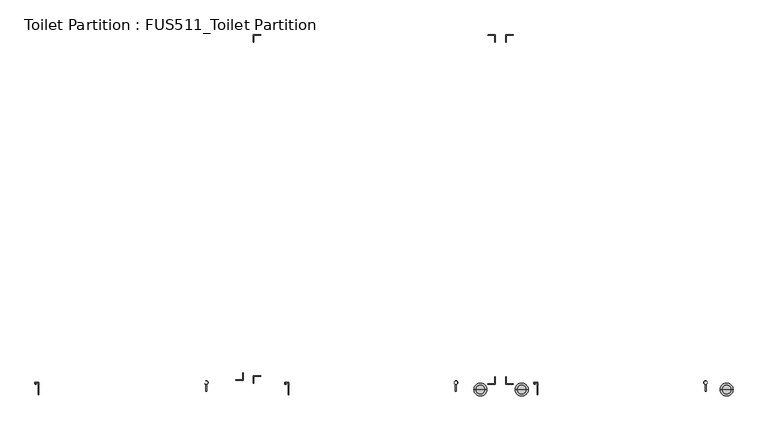
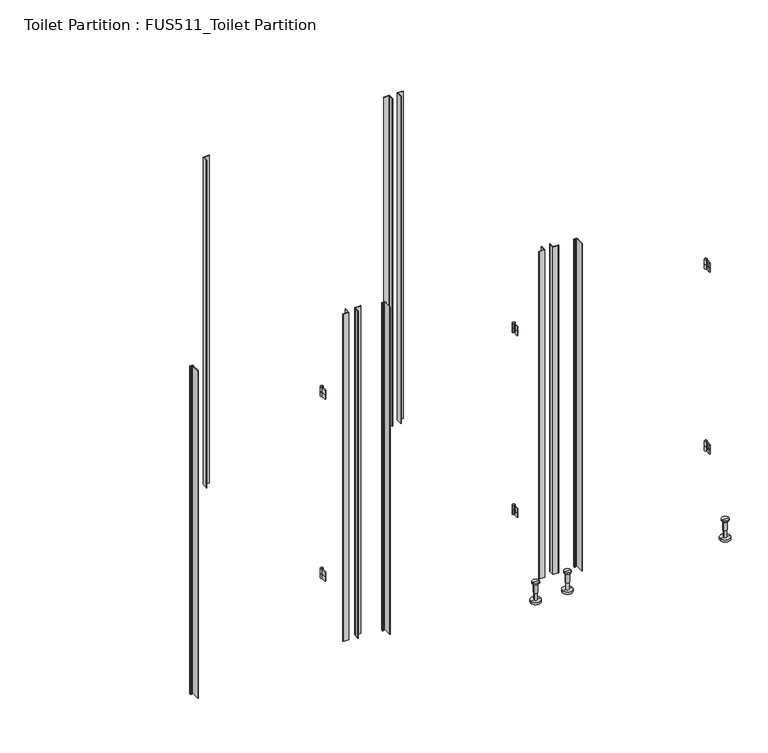
"""IFC4 building model written with IfcOpenShell, lengths in millimetres: furniture geometry, Toilet Partition : FUS511_Toilet Partition."""

from ifc_helpers import new_model, si_unit, point, frame, frame_2d, origin, place, context, project, spatial, polyline, circle_curve, trimmed, segment, composite_curve, outline, extrude, source, transform, mapped, element, save
from ifc_brep_helpers import plane_surface, cylinder_surface, advanced_brep


def toilet_partition_fus511_toilet_partition_2a8fb3a8(model_context):
    return source(origin(), model_context, "Body", "SolidModel", [
        extrude(outline(composite_curve([segment(trimmed(circle_curve(frame_2d((-483.6851629, 1892.2118377)), 1.0008364), [point((-483.6851629, 1893.2126742))], [point((-484.6859993, 1892.2118377))], True, "CARTESIAN"), True, "CONTINUOUS"), segment(polyline([(-484.6859993, 1892.2118377), (-484.6859993, 1865.1892547), (-485.6868357, 1865.1892547)]), True, "CONTINUOUS"), segment(trimmed(circle_curve(frame_2d((-485.6868357, 1866.1900911)), 1.0008364), [point((-485.6868357, 1865.1892547))], [point((-486.6876721, 1866.1900911))], False, "CARTESIAN"), True, "CONTINUOUS"), segment(polyline([(-486.6876721, 1866.1900911), (-486.6876721, 1895.214347), (-457.6634163, 1895.214347)]), True, "CONTINUOUS"), segment(trimmed(circle_curve(frame_2d((-457.6634163, 1894.2135106)), 1.0008364), [point((-457.6634163, 1895.214347))], [point((-456.6625798, 1894.2135106))], False, "CARTESIAN"), True, "CONTINUOUS"), segment(polyline([(-456.6625798, 1894.2135106), (-456.6625798, 1893.2126742), (-483.6851629, 1893.2126742)]), True, "CONTINUOUS")], self_intersect=False)), frame((0.0, 0.0, 100.0), z_axis=(0.0, 0.0, 1.0), x_axis=(1.0, 0.0, 0.0)), (0.0, 0.0, 1.0), 1800.0),
        extrude(outline(composite_curve([segment(polyline([(478.8769058, 1893.2126742), (451.8543227, 1893.2126742), (451.8543227, 1894.2135106)]), True, "CONTINUOUS"), segment(trimmed(circle_curve(frame_2d((452.8551591, 1894.2135106)), 1.0008364), [point((451.8543227, 1894.2135106))], [point((452.8551591, 1895.214347))], False, "CARTESIAN"), True, "CONTINUOUS"), segment(polyline([(452.8551591, 1895.214347), (481.879415, 1895.214347), (481.879415, 1866.1900911)]), True, "CONTINUOUS"), segment(trimmed(circle_curve(frame_2d((480.8785786, 1866.1900911)), 1.0008364), [point((481.879415, 1866.1900911))], [point((480.8785786, 1865.1892547))], False, "CARTESIAN"), True, "CONTINUOUS"), segment(polyline([(480.8785786, 1865.1892547), (479.8777422, 1865.1892547), (479.8777422, 1892.2118377)]), True, "CONTINUOUS"), segment(trimmed(circle_curve(frame_2d((478.8769058, 1892.2118377)), 1.0008364), [point((479.8777422, 1892.2118377))], [point((478.8769058, 1893.2126742))], True, "CARTESIAN"), True, "CONTINUOUS")], self_intersect=False)), frame((0.0, 0.0, 100.0), z_axis=(0.0, 0.0, 1.0), x_axis=(1.0, 0.0, 0.0)), (0.0, 0.0, 1.0), 1800.0),
        extrude(outline(composite_curve([segment(trimmed(circle_curve(frame_2d((525.8819242, 1892.2118377)), 1.0008364), [point((525.8819242, 1893.2126742))], [point((524.8810878, 1892.2118377))], True, "CARTESIAN"), True, "CONTINUOUS"), segment(polyline([(524.8810878, 1892.2118377), (524.8810878, 1865.1892547), (523.8802514, 1865.1892547)]), True, "CONTINUOUS"), segment(trimmed(circle_curve(frame_2d((523.8802514, 1866.1900911)), 1.0008364), [point((523.8802514, 1865.1892547))], [point((522.879415, 1866.1900911))], False, "CARTESIAN"), True, "CONTINUOUS"), segment(polyline([(522.879415, 1866.1900911), (522.879415, 1895.214347), (551.9036709, 1895.214347)]), True, "CONTINUOUS"), segment(trimmed(circle_curve(frame_2d((551.9036709, 1894.2135106)), 1.0008364), [point((551.9036709, 1895.214347))], [point((552.9045073, 1894.2135106))], False, "CARTESIAN"), True, "CONTINUOUS"), segment(polyline([(552.9045073, 1894.2135106), (552.9045073, 1893.2126742), (525.8819242, 1893.2126742)]), True, "CONTINUOUS")], self_intersect=False)), frame((0.0, 0.0, 100.0), z_axis=(0.0, 0.0, 1.0), x_axis=(1.0, 0.0, 0.0)), (0.0, 0.0, 1.0), 1800.0),
        extrude(outline(composite_curve([segment(trimmed(circle_curve(frame_2d((-530.6901814, 514.4572016)), 1.0008364), [point((-530.6901814, 513.4563652))], [point((-529.689345, 514.4572016))], True, "CARTESIAN"), True, "CONTINUOUS"), segment(polyline([(-529.689345, 514.4572016), (-529.689345, 541.4797847), (-528.6885085, 541.4797847)]), True, "CONTINUOUS"), segment(trimmed(circle_curve(frame_2d((-528.6885085, 540.4789483)), 1.0008364), [point((-528.6885085, 541.4797847))], [point((-527.6876721, 540.4789483))], False, "CARTESIAN"), True, "CONTINUOUS"), segment(polyline([(-527.6876721, 540.4789483), (-527.6876721, 511.4546924), (-556.711928, 511.4546924)]), True, "CONTINUOUS"), segment(trimmed(circle_curve(frame_2d((-556.711928, 512.4555288)), 1.0008364), [point((-556.711928, 511.4546924))], [point((-557.7127644, 512.4555288))], False, "CARTESIAN"), True, "CONTINUOUS"), segment(polyline([(-557.7127644, 512.4555288), (-557.7127644, 513.4563652), (-530.6901814, 513.4563652)]), True, "CONTINUOUS")], self_intersect=False)), frame((0.0, 0.0, 100.0), z_axis=(0.0, 0.0, 1.0), x_axis=(1.0, 0.0, 0.0)), (0.0, 0.0, 1.0), 1800.0),
        extrude(outline(composite_curve([segment(trimmed(circle_curve(frame_2d((-483.6851629, 527.0159753)), 1.0008364), [point((-483.6851629, 528.0168117))], [point((-484.6859993, 527.0159753))], True, "CARTESIAN"), True, "CONTINUOUS"), segment(polyline([(-484.6859993, 527.0159753), (-484.6859993, 499.9933923), (-485.6868357, 499.9933923)]), True, "CONTINUOUS"), segment(trimmed(circle_curve(frame_2d((-485.6868357, 500.9942287)), 1.0008364), [point((-485.6868357, 499.9933923))], [point((-486.6876721, 500.9942287))], False, "CARTESIAN"), True, "CONTINUOUS"), segment(polyline([(-486.6876721, 500.9942287), (-486.6876721, 530.0184846), (-457.6634163, 530.0184846)]), True, "CONTINUOUS"), segment(trimmed(circle_curve(frame_2d((-457.6634163, 529.0176481)), 1.0008364), [point((-457.6634163, 530.0184846))], [point((-456.6625798, 529.0176481))], False, "CARTESIAN"), True, "CONTINUOUS"), segment(polyline([(-456.6625798, 529.0176481), (-456.6625798, 528.0168117), (-483.6851629, 528.0168117)]), True, "CONTINUOUS")], self_intersect=False)), frame((0.0, 0.0, 100.0), z_axis=(0.0, 0.0, 1.0), x_axis=(1.0, 0.0, 0.0)), (0.0, 0.0, 1.0), 1800.0),
        extrude(outline(composite_curve([segment(trimmed(circle_curve(frame_2d((478.8769058, 498.2168562)), 1.0008364), [point((478.8769058, 497.2160198))], [point((479.8777422, 498.2168562))], True, "CARTESIAN"), True, "CONTINUOUS"), segment(polyline([(479.8777422, 498.2168562), (479.8777422, 525.2394393), (480.8785786, 525.2394393)]), True, "CONTINUOUS"), segment(trimmed(circle_curve(frame_2d((480.8785786, 524.2386029)), 1.0008364), [point((480.8785786, 525.2394393))], [point((481.879415, 524.2386029))], False, "CARTESIAN"), True, "CONTINUOUS"), segment(polyline([(481.879415, 524.2386029), (481.879415, 495.214347), (452.8551591, 495.214347)]), True, "CONTINUOUS"), segment(trimmed(circle_curve(frame_2d((452.8551591, 496.2151834)), 1.0008364), [point((452.8551591, 495.214347))], [point((451.8543227, 496.2151834))], False, "CARTESIAN"), True, "CONTINUOUS"), segment(polyline([(451.8543227, 496.2151834), (451.8543227, 497.2160198), (478.8769058, 497.2160198)]), True, "CONTINUOUS")], self_intersect=False)), frame((0.0, 0.0, 100.0), z_axis=(0.0, 0.0, 1.0), x_axis=(1.0, 0.0, 0.0)), (0.0, 0.0, 1.0), 1800.0),
        extrude(outline(composite_curve([segment(polyline([(525.8819242, 497.2160198), (552.9045073, 497.2160198), (552.9045073, 496.2151834)]), True, "CONTINUOUS"), segment(trimmed(circle_curve(frame_2d((551.9036709, 496.2151834)), 1.0008364), [point((552.9045073, 496.2151834))], [point((551.9036709, 495.214347))], False, "CARTESIAN"), True, "CONTINUOUS"), segment(polyline([(551.9036709, 495.214347), (522.879415, 495.214347), (522.879415, 524.2386029)]), True, "CONTINUOUS"), segment(trimmed(circle_curve(frame_2d((523.8802514, 524.2386029)), 1.0008364), [point((522.879415, 524.2386029))], [point((523.8802514, 525.2394393))], False, "CARTESIAN"), True, "CONTINUOUS"), segment(polyline([(523.8802514, 525.2394393), (524.8810878, 525.2394393), (524.8810878, 498.2168562)]), True, "CONTINUOUS"), segment(trimmed(circle_curve(frame_2d((525.8819242, 498.2168562)), 1.0008364), [point((524.8810878, 498.2168562))], [point((525.8819242, 497.2160198))], True, "CARTESIAN"), True, "CONTINUOUS")], self_intersect=False)), frame((0.0, 0.0, 100.0), z_axis=(0.0, 0.0, 1.0), x_axis=(1.0, 0.0, 0.0)), (0.0, 0.0, 1.0), 1800.0),
        extrude(outline(composite_curve([segment(trimmed(circle_curve(frame_2d((1322.6156791, 502.2850056)), 7.0), [point((1320.6156791, 495.5768017))], [point((1324.6156791, 495.5768017))], False, "CARTESIAN"), True, "CONTINUOUS"), segment(polyline([(1324.6156791, 495.5768017), (1324.6156791, 467.7850056), (1320.6156791, 467.7850056), (1320.6156791, 495.5768017)]), True, "CONTINUOUS")], self_intersect=False), holes=[composite_curve([segment(trimmed(circle_curve(frame_2d((1322.6156791, 502.2850056)), 6.0), [point((1316.6156791, 502.2850056))], [point((1328.6156791, 502.2850056))], True, "CARTESIAN"), True, "CONTINUOUS"), segment(trimmed(circle_curve(frame_2d((1322.6156791, 502.2850056)), 6.0), [point((1328.6156791, 502.2850056))], [point((1316.6156791, 502.2850056))], True, "CARTESIAN"), True, "CONTINUOUS")], self_intersect=False)]), frame((0.0, 0.0, 1525.0), z_axis=(0.0, 0.0, 1.0), x_axis=(1.0, 0.0, 0.0)), (0.0, 0.0, 1.0), 25.0),
        extrude(outline(composite_curve([segment(trimmed(circle_curve(frame_2d((1322.6156791, 502.2850056)), 7.0), [point((1320.6156791, 495.5768017))], [point((1324.6156791, 495.5768017))], False, "CARTESIAN"), True, "CONTINUOUS"), segment(polyline([(1324.6156791, 495.5768017), (1324.6156791, 467.7850056), (1320.6156791, 467.7850056), (1320.6156791, 495.5768017)]), True, "CONTINUOUS")], self_intersect=False), holes=[composite_curve([segment(trimmed(circle_curve(frame_2d((1322.6156791, 502.2850056)), 6.0), [point((1316.6156791, 502.2850056))], [point((1328.6156791, 502.2850056))], True, "CARTESIAN"), True, "CONTINUOUS"), segment(trimmed(circle_curve(frame_2d((1322.6156791, 502.2850056)), 6.0), [point((1328.6156791, 502.2850056))], [point((1316.6156791, 502.2850056))], True, "CARTESIAN"), True, "CONTINUOUS")], self_intersect=False)]), frame((0.0, 0.0, 1500.0), z_axis=(0.0, 0.0, 1.0), x_axis=(1.0, 0.0, 0.0)), (0.0, 0.0, 1.0), 25.0),
        extrude(outline(composite_curve([segment(trimmed(circle_curve(frame_2d((323.7360042, 502.2850056)), 7.0), [point((321.7360042, 495.5768017))], [point((325.7360042, 495.5768017))], False, "CARTESIAN"), True, "CONTINUOUS"), segment(polyline([(325.7360042, 495.5768017), (325.7360042, 467.7850056), (321.7360042, 467.7850056), (321.7360042, 495.5768017)]), True, "CONTINUOUS")], self_intersect=False), holes=[composite_curve([segment(trimmed(circle_curve(frame_2d((323.7360042, 502.2850056)), 6.0), [point((317.7360042, 502.2850056))], [point((329.7360042, 502.2850056))], True, "CARTESIAN"), True, "CONTINUOUS"), segment(trimmed(circle_curve(frame_2d((323.7360042, 502.2850056)), 6.0), [point((329.7360042, 502.2850056))], [point((317.7360042, 502.2850056))], True, "CARTESIAN"), True, "CONTINUOUS")], self_intersect=False)]), frame((0.0, 0.0, 1525.0), z_axis=(0.0, 0.0, 1.0), x_axis=(1.0, 0.0, 0.0)), (0.0, 0.0, 1.0), 25.0),
        extrude(outline(composite_curve([segment(trimmed(circle_curve(frame_2d((323.7360042, 502.2850056)), 7.0), [point((321.7360042, 495.5768017))], [point((325.7360042, 495.5768017))], False, "CARTESIAN"), True, "CONTINUOUS"), segment(polyline([(325.7360042, 495.5768017), (325.7360042, 467.7850056), (321.7360042, 467.7850056), (321.7360042, 495.5768017)]), True, "CONTINUOUS")], self_intersect=False), holes=[composite_curve([segment(trimmed(circle_curve(frame_2d((323.7360042, 502.2850056)), 6.0), [point((317.7360042, 502.2850056))], [point((329.7360042, 502.2850056))], True, "CARTESIAN"), True, "CONTINUOUS"), segment(trimmed(circle_curve(frame_2d((323.7360042, 502.2850056)), 6.0), [point((329.7360042, 502.2850056))], [point((317.7360042, 502.2850056))], True, "CARTESIAN"), True, "CONTINUOUS")], self_intersect=False)]), frame((0.0, 0.0, 1500.0), z_axis=(0.0, 0.0, 1.0), x_axis=(1.0, 0.0, 0.0)), (0.0, 0.0, 1.0), 25.0),
        extrude(outline(composite_curve([segment(trimmed(circle_curve(frame_2d((-675.1953266, 502.2850056)), 7.0), [point((-677.1953266, 495.5768017))], [point((-673.1953266, 495.5768017))], False, "CARTESIAN"), True, "CONTINUOUS"), segment(polyline([(-673.1953266, 495.5768017), (-673.1953266, 467.7850056), (-677.1953266, 467.7850056), (-677.1953266, 495.5768017)]), True, "CONTINUOUS")], self_intersect=False), holes=[composite_curve([segment(trimmed(circle_curve(frame_2d((-675.1953266, 502.2850056)), 6.0), [point((-681.1953266, 502.2850056))], [point((-669.1953266, 502.2850056))], True, "CARTESIAN"), True, "CONTINUOUS"), segment(trimmed(circle_curve(frame_2d((-675.1953266, 502.2850056)), 6.0), [point((-669.1953266, 502.2850056))], [point((-681.1953266, 502.2850056))], True, "CARTESIAN"), True, "CONTINUOUS")], self_intersect=False)]), frame((0.0, 0.0, 1525.0), z_axis=(0.0, 0.0, 1.0), x_axis=(1.0, 0.0, 0.0)), (0.0, 0.0, 1.0), 25.0),
        extrude(outline(composite_curve([segment(trimmed(circle_curve(frame_2d((-675.1953266, 502.2850056)), 7.0), [point((-677.1953266, 495.5768017))], [point((-673.1953266, 495.5768017))], False, "CARTESIAN"), True, "CONTINUOUS"), segment(polyline([(-673.1953266, 495.5768017), (-673.1953266, 467.7850056), (-677.1953266, 467.7850056), (-677.1953266, 495.5768017)]), True, "CONTINUOUS")], self_intersect=False), holes=[composite_curve([segment(trimmed(circle_curve(frame_2d((-675.1953266, 502.2850056)), 6.0), [point((-681.1953266, 502.2850056))], [point((-669.1953266, 502.2850056))], True, "CARTESIAN"), True, "CONTINUOUS"), segment(trimmed(circle_curve(frame_2d((-675.1953266, 502.2850056)), 6.0), [point((-669.1953266, 502.2850056))], [point((-681.1953266, 502.2850056))], True, "CARTESIAN"), True, "CONTINUOUS")], self_intersect=False)]), frame((0.0, 0.0, 1500.0), z_axis=(0.0, 0.0, 1.0), x_axis=(1.0, 0.0, 0.0)), (0.0, 0.0, 1.0), 25.0),
        extrude(outline(composite_curve([segment(trimmed(circle_curve(frame_2d((1322.6156791, 502.2850056)), 7.0), [point((1320.6156791, 495.5768017))], [point((1324.6156791, 495.5768017))], False, "CARTESIAN"), True, "CONTINUOUS"), segment(polyline([(1324.6156791, 495.5768017), (1324.6156791, 467.7850056), (1320.6156791, 467.7850056), (1320.6156791, 495.5768017)]), True, "CONTINUOUS")], self_intersect=False), holes=[composite_curve([segment(trimmed(circle_curve(frame_2d((1322.6156791, 502.2850056)), 6.0), [point((1316.6156791, 502.2850056))], [point((1328.6156791, 502.2850056))], True, "CARTESIAN"), True, "CONTINUOUS"), segment(trimmed(circle_curve(frame_2d((1322.6156791, 502.2850056)), 6.0), [point((1328.6156791, 502.2850056))], [point((1316.6156791, 502.2850056))], True, "CARTESIAN"), True, "CONTINUOUS")], self_intersect=False)]), frame((0.0, 0.0, 525.0), z_axis=(0.0, 0.0, 1.0), x_axis=(1.0, 0.0, 0.0)), (0.0, 0.0, 1.0), 25.0),
        extrude(outline(composite_curve([segment(trimmed(circle_curve(frame_2d((1322.6156791, 502.2850056)), 7.0), [point((1320.6156791, 495.5768017))], [point((1324.6156791, 495.5768017))], False, "CARTESIAN"), True, "CONTINUOUS"), segment(polyline([(1324.6156791, 495.5768017), (1324.6156791, 467.7850056), (1320.6156791, 467.7850056), (1320.6156791, 495.5768017)]), True, "CONTINUOUS")], self_intersect=False), holes=[composite_curve([segment(trimmed(circle_curve(frame_2d((1322.6156791, 502.2850056)), 6.0), [point((1316.6156791, 502.2850056))], [point((1328.6156791, 502.2850056))], True, "CARTESIAN"), True, "CONTINUOUS"), segment(trimmed(circle_curve(frame_2d((1322.6156791, 502.2850056)), 6.0), [point((1328.6156791, 502.2850056))], [point((1316.6156791, 502.2850056))], True, "CARTESIAN"), True, "CONTINUOUS")], self_intersect=False)]), frame((0.0, 0.0, 500.0), z_axis=(0.0, 0.0, 1.0), x_axis=(1.0, 0.0, 0.0)), (0.0, 0.0, 1.0), 25.0),
        extrude(outline(composite_curve([segment(trimmed(circle_curve(frame_2d((323.7360042, 502.2850056)), 7.0), [point((321.7360042, 495.5768017))], [point((325.7360042, 495.5768017))], False, "CARTESIAN"), True, "CONTINUOUS"), segment(polyline([(325.7360042, 495.5768017), (325.7360042, 467.7850056), (321.7360042, 467.7850056), (321.7360042, 495.5768017)]), True, "CONTINUOUS")], self_intersect=False), holes=[composite_curve([segment(trimmed(circle_curve(frame_2d((323.7360042, 502.2850056)), 6.0), [point((317.7360042, 502.2850056))], [point((329.7360042, 502.2850056))], True, "CARTESIAN"), True, "CONTINUOUS"), segment(trimmed(circle_curve(frame_2d((323.7360042, 502.2850056)), 6.0), [point((329.7360042, 502.2850056))], [point((317.7360042, 502.2850056))], True, "CARTESIAN"), True, "CONTINUOUS")], self_intersect=False)]), frame((0.0, 0.0, 525.0), z_axis=(0.0, 0.0, 1.0), x_axis=(1.0, 0.0, 0.0)), (0.0, 0.0, 1.0), 25.0),
        extrude(outline(composite_curve([segment(trimmed(circle_curve(frame_2d((323.7360042, 502.2850056)), 7.0), [point((321.7360042, 495.5768017))], [point((325.7360042, 495.5768017))], False, "CARTESIAN"), True, "CONTINUOUS"), segment(polyline([(325.7360042, 495.5768017), (325.7360042, 467.7850056), (321.7360042, 467.7850056), (321.7360042, 495.5768017)]), True, "CONTINUOUS")], self_intersect=False), holes=[composite_curve([segment(trimmed(circle_curve(frame_2d((323.7360042, 502.2850056)), 6.0), [point((317.7360042, 502.2850056))], [point((329.7360042, 502.2850056))], True, "CARTESIAN"), True, "CONTINUOUS"), segment(trimmed(circle_curve(frame_2d((323.7360042, 502.2850056)), 6.0), [point((329.7360042, 502.2850056))], [point((317.7360042, 502.2850056))], True, "CARTESIAN"), True, "CONTINUOUS")], self_intersect=False)]), frame((0.0, 0.0, 500.0), z_axis=(0.0, 0.0, 1.0), x_axis=(1.0, 0.0, 0.0)), (0.0, 0.0, 1.0), 25.0),
        extrude(outline(composite_curve([segment(trimmed(circle_curve(frame_2d((-675.1953266, 502.2850056)), 7.0), [point((-677.1953266, 495.5768017))], [point((-673.1953266, 495.5768017))], False, "CARTESIAN"), True, "CONTINUOUS"), segment(polyline([(-673.1953266, 495.5768017), (-673.1953266, 467.7850056), (-677.1953266, 467.7850056), (-677.1953266, 495.5768017)]), True, "CONTINUOUS")], self_intersect=False), holes=[composite_curve([segment(trimmed(circle_curve(frame_2d((-675.1953266, 502.2850056)), 6.0), [point((-681.1953266, 502.2850056))], [point((-669.1953266, 502.2850056))], True, "CARTESIAN"), True, "CONTINUOUS"), segment(trimmed(circle_curve(frame_2d((-675.1953266, 502.2850056)), 6.0), [point((-669.1953266, 502.2850056))], [point((-681.1953266, 502.2850056))], True, "CARTESIAN"), True, "CONTINUOUS")], self_intersect=False)]), frame((0.0, 0.0, 525.0), z_axis=(0.0, 0.0, 1.0), x_axis=(1.0, 0.0, 0.0)), (0.0, 0.0, 1.0), 25.0),
        extrude(outline(composite_curve([segment(trimmed(circle_curve(frame_2d((-675.1953266, 502.2850056)), 7.0), [point((-677.1953266, 495.5768017))], [point((-673.1953266, 495.5768017))], False, "CARTESIAN"), True, "CONTINUOUS"), segment(polyline([(-673.1953266, 495.5768017), (-673.1953266, 467.7850056), (-677.1953266, 467.7850056), (-677.1953266, 495.5768017)]), True, "CONTINUOUS")], self_intersect=False), holes=[composite_curve([segment(trimmed(circle_curve(frame_2d((-675.1953266, 502.2850056)), 6.0), [point((-681.1953266, 502.2850056))], [point((-669.1953266, 502.2850056))], True, "CARTESIAN"), True, "CONTINUOUS"), segment(trimmed(circle_curve(frame_2d((-675.1953266, 502.2850056)), 6.0), [point((-669.1953266, 502.2850056))], [point((-681.1953266, 502.2850056))], True, "CARTESIAN"), True, "CONTINUOUS")], self_intersect=False)]), frame((0.0, 0.0, 500.0), z_axis=(0.0, 0.0, 1.0), x_axis=(1.0, 0.0, 0.0)), (0.0, 0.0, 1.0), 25.0),
        extrude(outline(polyline([(635.6294456, 503.4888254), (651.4228263, 503.4888254), (651.4228263, 499.4012527), (653.8741408, 495.1554513), (652.7343518, 495.1554513), (651.4228263, 497.4270801), (651.4228263, 454.1345106), (649.4486537, 454.1345106), (649.4486537, 501.5146528), (645.826099, 501.5146528), (641.7674724, 497.0112968), (640.6276833, 497.0112968), (644.6863099, 501.5146528), (636.6165319, 501.5146528), (636.6165319, 497.8847941), (638.0262016, 497.8847941), (638.0262016, 497.0402783), (635.6294456, 497.0402783), (635.6294456, 503.4888254)])), frame((0.0, 0.0, 100.0), z_axis=(0.0, 0.0, 1.0), x_axis=(1.0, 0.0, 0.0)), (0.0, 0.0, 1.0), 1800.0),
        extrude(outline(composite_curve([segment(polyline([(640.8337808, 495.214347), (637.7985331, 495.214347)]), True, "CONTINUOUS"), segment(trimmed(circle_curve(frame_2d((637.7985331, 496.004016)), 0.789669), [point((637.7985331, 495.214347))], [point((637.0088641, 496.004016))], False, "CARTESIAN"), True, "CONTINUOUS"), segment(polyline([(637.0088641, 496.004016), (637.0088641, 496.8402783), (638.1566952, 496.8402783)]), True, "CONTINUOUS"), segment(trimmed(circle_curve(frame_2d((637.5137871, 497.4916495)), 0.9152132), [point((638.1566952, 496.8402783))], [point((638.1251074, 498.1727534))], True, "CARTESIAN"), True, "CONTINUOUS"), segment(trimmed(circle_curve(frame_2d((638.4034381, 498.4828563)), 0.4166915), [point((638.1251074, 498.1727534))], [point((638.2496827, 498.870143))], False, "CARTESIAN"), True, "CONTINUOUS"), segment(trimmed(circle_curve(frame_2d((639.3215602, 496.1702449)), 2.9048875), [point((638.2496827, 498.870143))], [point((640.4174512, 498.8604854))], False, "CARTESIAN"), True, "CONTINUOUS"), segment(trimmed(circle_curve(frame_2d((640.2672492, 498.4917631)), 0.3981417), [point((640.4174512, 498.8604854))], [point((640.5253128, 498.1885801))], False, "CARTESIAN"), True, "CONTINUOUS"), segment(trimmed(circle_curve(frame_2d((641.1185268, 497.4916495)), 0.9152132), [point((640.5253128, 498.1885801))], [point((640.4756187, 496.8402783))], True, "CARTESIAN"), True, "CONTINUOUS"), segment(polyline([(640.4756187, 496.8402783), (641.6234499, 496.8402783), (641.6234499, 496.004016)]), True, "CONTINUOUS"), segment(trimmed(circle_curve(frame_2d((640.8337808, 496.004016)), 0.789669), [point((641.6234499, 496.004016))], [point((640.8337808, 495.214347))], False, "CARTESIAN"), True, "CONTINUOUS")], self_intersect=False)), frame((0.0, 0.0, 100.0), z_axis=(0.0, 0.0, 1.0), x_axis=(1.0, 0.0, 0.0)), (0.0, 0.0, 1.0), 1800.0),
        extrude(outline(polyline([(-362.0057179, 503.4888254), (-346.2123372, 503.4888254), (-346.2123372, 499.4012527), (-343.7610226, 495.1554513), (-344.9008117, 495.1554513), (-346.2123372, 497.4270801), (-346.2123372, 454.1345106), (-348.1865098, 454.1345106), (-348.1865098, 501.5146528), (-351.8090644, 501.5146528), (-355.8676911, 497.0112968), (-357.0074802, 497.0112968), (-352.9488535, 501.5146528), (-361.0186316, 501.5146528), (-361.0186316, 497.8847941), (-359.6089619, 497.8847941), (-359.6089619, 497.0402783), (-362.0057179, 497.0402783), (-362.0057179, 503.4888254)])), frame((0.0, 0.0, 100.0), z_axis=(0.0, 0.0, 1.0), x_axis=(1.0, 0.0, 0.0)), (0.0, 0.0, 1.0), 1800.0),
        extrude(outline(composite_curve([segment(polyline([(-356.8013826, 495.214347), (-359.8366303, 495.214347)]), True, "CONTINUOUS"), segment(trimmed(circle_curve(frame_2d((-359.8366303, 496.004016)), 0.789669), [point((-359.8366303, 495.214347))], [point((-360.6262994, 496.004016))], False, "CARTESIAN"), True, "CONTINUOUS"), segment(polyline([(-360.6262994, 496.004016), (-360.6262994, 496.8402783), (-359.4784683, 496.8402783)]), True, "CONTINUOUS"), segment(trimmed(circle_curve(frame_2d((-360.1213764, 497.4916495)), 0.9152132), [point((-359.4784683, 496.8402783))], [point((-359.510056, 498.1727534))], True, "CARTESIAN"), True, "CONTINUOUS"), segment(trimmed(circle_curve(frame_2d((-359.2317253, 498.4828563)), 0.4166915), [point((-359.510056, 498.1727534))], [point((-359.3854807, 498.870143))], False, "CARTESIAN"), True, "CONTINUOUS"), segment(trimmed(circle_curve(frame_2d((-358.3136033, 496.1702449)), 2.9048875), [point((-359.3854807, 498.870143))], [point((-357.2177122, 498.8604854))], False, "CARTESIAN"), True, "CONTINUOUS"), segment(trimmed(circle_curve(frame_2d((-357.3679142, 498.4917631)), 0.3981417), [point((-357.2177122, 498.8604854))], [point((-357.1098506, 498.1885801))], False, "CARTESIAN"), True, "CONTINUOUS"), segment(trimmed(circle_curve(frame_2d((-356.5166366, 497.4916495)), 0.9152132), [point((-357.1098506, 498.1885801))], [point((-357.1595447, 496.8402783))], True, "CARTESIAN"), True, "CONTINUOUS"), segment(polyline([(-357.1595447, 496.8402783), (-356.0117136, 496.8402783), (-356.0117136, 496.004016)]), True, "CONTINUOUS"), segment(trimmed(circle_curve(frame_2d((-356.8013826, 496.004016)), 0.789669), [point((-356.0117136, 496.004016))], [point((-356.8013826, 495.214347))], False, "CARTESIAN"), True, "CONTINUOUS")], self_intersect=False)), frame((0.0, 0.0, 100.0), z_axis=(0.0, 0.0, 1.0), x_axis=(1.0, 0.0, 0.0)), (0.0, 0.0, 1.0), 1800.0),
        extrude(outline(polyline([(-1360.9370525, 503.4888254), (-1345.1436718, 503.4888254), (-1345.1436718, 499.4012527), (-1342.6923572, 495.1554513), (-1343.8321463, 495.1554513), (-1345.1436718, 497.4270801), (-1345.1436718, 454.1345106), (-1347.1178444, 454.1345106), (-1347.1178444, 501.5146528), (-1350.740399, 501.5146528), (-1354.7990257, 497.0112968), (-1355.9388148, 497.0112968), (-1351.8801881, 501.5146528), (-1359.9499662, 501.5146528), (-1359.9499662, 497.8847941), (-1358.5402965, 497.8847941), (-1358.5402965, 497.0402783), (-1360.9370525, 497.0402783), (-1360.9370525, 503.4888254)])), frame((0.0, 0.0, 100.0), z_axis=(0.0, 0.0, 1.0), x_axis=(1.0, 0.0, 0.0)), (0.0, 0.0, 1.0), 1800.0),
        extrude(outline(composite_curve([segment(polyline([(-1355.7327172, 495.214347), (-1358.7679649, 495.214347)]), True, "CONTINUOUS"), segment(trimmed(circle_curve(frame_2d((-1358.7679649, 496.004016)), 0.789669), [point((-1358.7679649, 495.214347))], [point((-1359.557634, 496.004016))], False, "CARTESIAN"), True, "CONTINUOUS"), segment(polyline([(-1359.557634, 496.004016), (-1359.557634, 496.8402783), (-1358.4098029, 496.8402783)]), True, "CONTINUOUS"), segment(trimmed(circle_curve(frame_2d((-1359.052711, 497.4916495)), 0.9152132), [point((-1358.4098029, 496.8402783))], [point((-1358.4413906, 498.1727534))], True, "CARTESIAN"), True, "CONTINUOUS"), segment(trimmed(circle_curve(frame_2d((-1358.1630599, 498.4828563)), 0.4166915), [point((-1358.4413906, 498.1727534))], [point((-1358.3168153, 498.870143))], False, "CARTESIAN"), True, "CONTINUOUS"), segment(trimmed(circle_curve(frame_2d((-1357.2449378, 496.1702449)), 2.9048875), [point((-1358.3168153, 498.870143))], [point((-1356.1490468, 498.8604854))], False, "CARTESIAN"), True, "CONTINUOUS"), segment(trimmed(circle_curve(frame_2d((-1356.2992488, 498.4917631)), 0.3981417), [point((-1356.1490468, 498.8604854))], [point((-1356.0411852, 498.1885801))], False, "CARTESIAN"), True, "CONTINUOUS"), segment(trimmed(circle_curve(frame_2d((-1355.4479712, 497.4916495)), 0.9152132), [point((-1356.0411852, 498.1885801))], [point((-1356.0908793, 496.8402783))], True, "CARTESIAN"), True, "CONTINUOUS"), segment(polyline([(-1356.0908793, 496.8402783), (-1354.9430482, 496.8402783), (-1354.9430482, 496.004016)]), True, "CONTINUOUS"), segment(trimmed(circle_curve(frame_2d((-1355.7327172, 496.004016)), 0.789669), [point((-1354.9430482, 496.004016))], [point((-1355.7327172, 495.214347))], False, "CARTESIAN"), True, "CONTINUOUS")], self_intersect=False)), frame((0.0, 0.0, 100.0), z_axis=(0.0, 0.0, 1.0), x_axis=(1.0, 0.0, 0.0)), (0.0, 0.0, 1.0), 1800.0),
        advanced_brep(
        [(1391.087395, 474.714347, 104.1461397), (1422.3312369, 474.714347, 104.1461397), (1422.3312369, 474.714347, 101.0217555), (1391.087395, 474.714347, 101.0217555), (1380.6727811, 474.714347, 0.0), (1432.7458509, 474.714347, 0.0), (1406.709316, 474.714347, 0.0), (1380.6727811, 474.714347, 10.414614), (1432.7458509, 474.714347, 10.414614), (1398.8983555, 474.714347, 10.414614), (1414.5202765, 474.714347, 10.414614), (1398.8983555, 474.714347, 52.0730698), (1414.5202765, 474.714347, 52.0730698), (1396.294702, 474.714347, 52.0730698), (1417.1239299, 474.714347, 52.0730698), (1396.294702, 474.714347, 101.0217555), (1417.1239299, 474.714347, 101.0217555), (1389.0044722, 474.714347, 104.1461397), (1424.4141597, 474.714347, 104.1461397), (1389.0044722, 474.714347, 110.394908), (1424.4141597, 474.714347, 110.394908), (1406.709316, 474.714347, 110.394908)],
        [
            (0, 1, circle_curve(frame((1406.709316, 474.714347, 104.1461397), z_axis=(0.0, 0.0, -1.0), x_axis=(1.0, 0.0, 0.0)), 15.6219209)),
            (1, 2),
            (2, 3, circle_curve(frame((1406.709316, 474.714347, 101.0217555), z_axis=(0.0, 0.0, 1.0), x_axis=(1.0, 0.0, 0.0)), 15.6219209)),
            (3, 0),
            (1, 0, circle_curve(frame((1406.709316, 474.714347, 104.1461397), z_axis=(0.0, 0.0, -1.0), x_axis=(1.0, 0.0, 0.0)), 15.6219209)),
            (3, 2, circle_curve(frame((1406.709316, 474.714347, 101.0217555), z_axis=(0.0, 0.0, 1.0), x_axis=(1.0, 0.0, 0.0)), 15.6219209)),
            (4, 5, circle_curve(frame((1406.709316, 474.714347, 0.0), z_axis=(0.0, 0.0, -1.0), x_axis=(1.0, 0.0, 0.0)), 26.0365349)),
            (5, 6),
            (6, 4),
            (5, 4, circle_curve(frame((1406.709316, 474.714347, 0.0), z_axis=(0.0, 0.0, -1.0), x_axis=(1.0, 0.0, 0.0)), 26.0365349)),
            (7, 8, circle_curve(frame((1406.709316, 474.714347, 10.414614), z_axis=(0.0, 0.0, -1.0), x_axis=(1.0, 0.0, 0.0)), 26.0365349)),
            (8, 5),
            (4, 7),
            (8, 7, circle_curve(frame((1406.709316, 474.714347, 10.414614), z_axis=(0.0, 0.0, -1.0), x_axis=(1.0, 0.0, 0.0)), 26.0365349)),
            (9, 10, circle_curve(frame((1406.709316, 474.714347, 10.414614), z_axis=(0.0, 0.0, -1.0), x_axis=(1.0, 0.0, 0.0)), 7.8109605)),
            (10, 8),
            (7, 9),
            (10, 9, circle_curve(frame((1406.709316, 474.714347, 10.414614), z_axis=(0.0, 0.0, -1.0), x_axis=(1.0, 0.0, 0.0)), 7.8109605)),
            (11, 12, circle_curve(frame((1406.709316, 474.714347, 52.0730698), z_axis=(0.0, 0.0, -1.0), x_axis=(1.0, 0.0, 0.0)), 7.8109605)),
            (12, 10),
            (9, 11),
            (12, 11, circle_curve(frame((1406.709316, 474.714347, 52.0730698), z_axis=(0.0, 0.0, -1.0), x_axis=(1.0, 0.0, 0.0)), 7.8109605)),
            (13, 14, circle_curve(frame((1406.709316, 474.714347, 52.0730698), z_axis=(0.0, 0.0, -1.0), x_axis=(1.0, 0.0, 0.0)), 10.414614)),
            (14, 12),
            (11, 13),
            (14, 13, circle_curve(frame((1406.709316, 474.714347, 52.0730698), z_axis=(0.0, 0.0, -1.0), x_axis=(1.0, 0.0, 0.0)), 10.414614)),
            (15, 16, circle_curve(frame((1406.709316, 474.714347, 101.0217555), z_axis=(0.0, 0.0, -1.0), x_axis=(1.0, 0.0, 0.0)), 10.414614)),
            (16, 14),
            (13, 15),
            (16, 15, circle_curve(frame((1406.709316, 474.714347, 101.0217555), z_axis=(0.0, 0.0, -1.0), x_axis=(1.0, 0.0, 0.0)), 10.414614)),
            (2, 16),
            (15, 3),
            (17, 18, circle_curve(frame((1406.709316, 474.714347, 104.1461397), z_axis=(0.0, 0.0, -1.0), x_axis=(1.0, 0.0, 0.0)), 17.7048437)),
            (18, 1),
            (0, 17),
            (18, 17, circle_curve(frame((1406.709316, 474.714347, 104.1461397), z_axis=(0.0, 0.0, -1.0), x_axis=(1.0, 0.0, 0.0)), 17.7048437)),
            (19, 20, circle_curve(frame((1406.709316, 474.714347, 110.394908), z_axis=(0.0, 0.0, -1.0), x_axis=(1.0, 0.0, 0.0)), 17.7048437)),
            (20, 18),
            (17, 19),
            (20, 19, circle_curve(frame((1406.709316, 474.714347, 110.394908), z_axis=(0.0, 0.0, -1.0), x_axis=(1.0, 0.0, 0.0)), 17.7048437)),
            (21, 20),
            (19, 21),
        ],
        [
            cylinder_surface(frame((1406.709316, 474.714347, 190.0), z_axis=(0.0, 0.0, 1.0), x_axis=(1.0, 0.0, 0.0)), 15.6219209),
            plane_surface(frame((1406.709316, 474.714347, 0.0), z_axis=(0.0, 0.0, -1.0), x_axis=(1.0, 0.0, 0.0))),
            cylinder_surface(frame((1406.709316, 474.714347, 190.0), z_axis=(0.0, 0.0, 1.0), x_axis=(1.0, 0.0, 0.0)), 26.0365349),
            plane_surface(frame((1406.709316, 474.714347, 10.414614), z_axis=(0.0, 0.0, 1.0), x_axis=(1.0, 0.0, 0.0))),
            cylinder_surface(frame((1406.709316, 474.714347, 190.0), z_axis=(0.0, 0.0, 1.0), x_axis=(1.0, 0.0, 0.0)), 7.8109605),
            plane_surface(frame((1406.709316, 474.714347, 52.0730698), z_axis=(0.0, 0.0, -1.0), x_axis=(1.0, 0.0, 0.0))),
            cylinder_surface(frame((1406.709316, 474.714347, 190.0), z_axis=(0.0, 0.0, 1.0), x_axis=(1.0, 0.0, 0.0)), 10.414614),
            plane_surface(frame((1406.709316, 474.714347, 101.0217555), z_axis=(0.0, 0.0, -1.0), x_axis=(1.0, 0.0, 0.0))),
            plane_surface(frame((1406.709316, 474.714347, 104.1461397), z_axis=(0.0, 0.0, -1.0), x_axis=(1.0, 0.0, 0.0))),
            cylinder_surface(frame((1406.709316, 474.714347, 190.0), z_axis=(0.0, 0.0, 1.0), x_axis=(1.0, 0.0, 0.0)), 17.7048437),
            plane_surface(frame((1406.709316, 474.714347, 110.394908), z_axis=(0.0, 0.0, 1.0), x_axis=(1.0, 0.0, 0.0))),
        ],
        [
            (0, [[1, 2, 3, 4]]),
            (0, [[5, -4, 6, -2]]),
            (1, [[7, 8, 9]]),
            (1, [[10, -9, -8]]),
            (2, [[11, 12, -7, 13]]),
            (2, [[14, -13, -10, -12]]),
            (3, [[15, 16, -11, 17]]),
            (3, [[18, -17, -14, -16]]),
            (4, [[19, 20, -15, 21]]),
            (4, [[22, -21, -18, -20]]),
            (5, [[23, 24, -19, 25]]),
            (5, [[26, -25, -22, -24]]),
            (6, [[27, 28, -23, 29]]),
            (6, [[30, -29, -26, -28]]),
            (7, [[-3, 31, -27, 32]]),
            (7, [[-6, -32, -30, -31]]),
            (8, [[33, 34, -1, 35]]),
            (8, [[36, -35, -5, -34]]),
            (9, [[37, 38, -33, 39]]),
            (9, [[40, -39, -36, -38]]),
            (10, [[41, -37, 42]]),
            (10, [[-42, -40, -41]]),
        ],
    ),
        advanced_brep(
        [(571.087395, 474.714347, 104.1461397), (602.3312369, 474.714347, 104.1461397), (602.3312369, 474.714347, 101.0217555), (571.087395, 474.714347, 101.0217555), (560.6727811, 474.714347, 0.0), (612.7458509, 474.714347, 0.0), (586.709316, 474.714347, 0.0), (560.6727811, 474.714347, 10.414614), (612.7458509, 474.714347, 10.414614), (578.8983555, 474.714347, 10.414614), (594.5202765, 474.714347, 10.414614), (578.8983555, 474.714347, 52.0730698), (594.5202765, 474.714347, 52.0730698), (576.294702, 474.714347, 52.0730698), (597.1239299, 474.714347, 52.0730698), (576.294702, 474.714347, 101.0217555), (597.1239299, 474.714347, 101.0217555), (569.0044722, 474.714347, 104.1461397), (604.4141597, 474.714347, 104.1461397), (569.0044722, 474.714347, 110.394908), (604.4141597, 474.714347, 110.394908), (586.709316, 474.714347, 110.394908)],
        [
            (0, 1, circle_curve(frame((586.709316, 474.714347, 104.1461397), z_axis=(0.0, 0.0, -1.0), x_axis=(1.0, 0.0, 0.0)), 15.6219209)),
            (1, 2),
            (2, 3, circle_curve(frame((586.709316, 474.714347, 101.0217555), z_axis=(0.0, 0.0, 1.0), x_axis=(1.0, 0.0, 0.0)), 15.6219209)),
            (3, 0),
            (1, 0, circle_curve(frame((586.709316, 474.714347, 104.1461397), z_axis=(0.0, 0.0, -1.0), x_axis=(1.0, 0.0, 0.0)), 15.6219209)),
            (3, 2, circle_curve(frame((586.709316, 474.714347, 101.0217555), z_axis=(0.0, 0.0, 1.0), x_axis=(1.0, 0.0, 0.0)), 15.6219209)),
            (4, 5, circle_curve(frame((586.709316, 474.714347, 0.0), z_axis=(0.0, 0.0, -1.0), x_axis=(1.0, 0.0, 0.0)), 26.0365349)),
            (5, 6),
            (6, 4),
            (5, 4, circle_curve(frame((586.709316, 474.714347, 0.0), z_axis=(0.0, 0.0, -1.0), x_axis=(1.0, 0.0, 0.0)), 26.0365349)),
            (7, 8, circle_curve(frame((586.709316, 474.714347, 10.414614), z_axis=(0.0, 0.0, -1.0), x_axis=(1.0, 0.0, 0.0)), 26.0365349)),
            (8, 5),
            (4, 7),
            (8, 7, circle_curve(frame((586.709316, 474.714347, 10.414614), z_axis=(0.0, 0.0, -1.0), x_axis=(1.0, 0.0, 0.0)), 26.0365349)),
            (9, 10, circle_curve(frame((586.709316, 474.714347, 10.414614), z_axis=(0.0, 0.0, -1.0), x_axis=(1.0, 0.0, 0.0)), 7.8109605)),
            (10, 8),
            (7, 9),
            (10, 9, circle_curve(frame((586.709316, 474.714347, 10.414614), z_axis=(0.0, 0.0, -1.0), x_axis=(1.0, 0.0, 0.0)), 7.8109605)),
            (11, 12, circle_curve(frame((586.709316, 474.714347, 52.0730698), z_axis=(0.0, 0.0, -1.0), x_axis=(1.0, 0.0, 0.0)), 7.8109605)),
            (12, 10),
            (9, 11),
            (12, 11, circle_curve(frame((586.709316, 474.714347, 52.0730698), z_axis=(0.0, 0.0, -1.0), x_axis=(1.0, 0.0, 0.0)), 7.8109605)),
            (13, 14, circle_curve(frame((586.709316, 474.714347, 52.0730698), z_axis=(0.0, 0.0, -1.0), x_axis=(1.0, 0.0, 0.0)), 10.414614)),
            (14, 12),
            (11, 13),
            (14, 13, circle_curve(frame((586.709316, 474.714347, 52.0730698), z_axis=(0.0, 0.0, -1.0), x_axis=(1.0, 0.0, 0.0)), 10.414614)),
            (15, 16, circle_curve(frame((586.709316, 474.714347, 101.0217555), z_axis=(0.0, 0.0, -1.0), x_axis=(1.0, 0.0, 0.0)), 10.414614)),
            (16, 14),
            (13, 15),
            (16, 15, circle_curve(frame((586.709316, 474.714347, 101.0217555), z_axis=(0.0, 0.0, -1.0), x_axis=(1.0, 0.0, 0.0)), 10.414614)),
            (2, 16),
            (15, 3),
            (17, 18, circle_curve(frame((586.709316, 474.714347, 104.1461397), z_axis=(0.0, 0.0, -1.0), x_axis=(1.0, 0.0, 0.0)), 17.7048437)),
            (18, 1),
            (0, 17),
            (18, 17, circle_curve(frame((586.709316, 474.714347, 104.1461397), z_axis=(0.0, 0.0, -1.0), x_axis=(1.0, 0.0, 0.0)), 17.7048437)),
            (19, 20, circle_curve(frame((586.709316, 474.714347, 110.394908), z_axis=(0.0, 0.0, -1.0), x_axis=(1.0, 0.0, 0.0)), 17.7048437)),
            (20, 18),
            (17, 19),
            (20, 19, circle_curve(frame((586.709316, 474.714347, 110.394908), z_axis=(0.0, 0.0, -1.0), x_axis=(1.0, 0.0, 0.0)), 17.7048437)),
            (21, 20),
            (19, 21),
        ],
        [
            cylinder_surface(frame((586.709316, 474.714347, 190.0), z_axis=(0.0, 0.0, 1.0), x_axis=(1.0, 0.0, 0.0)), 15.6219209),
            plane_surface(frame((586.709316, 474.714347, 0.0), z_axis=(0.0, 0.0, -1.0), x_axis=(1.0, 0.0, 0.0))),
            cylinder_surface(frame((586.709316, 474.714347, 190.0), z_axis=(0.0, 0.0, 1.0), x_axis=(1.0, 0.0, 0.0)), 26.0365349),
            plane_surface(frame((586.709316, 474.714347, 10.414614), z_axis=(0.0, 0.0, 1.0), x_axis=(1.0, 0.0, 0.0))),
            cylinder_surface(frame((586.709316, 474.714347, 190.0), z_axis=(0.0, 0.0, 1.0), x_axis=(1.0, 0.0, 0.0)), 7.8109605),
            plane_surface(frame((586.709316, 474.714347, 52.0730698), z_axis=(0.0, 0.0, -1.0), x_axis=(1.0, 0.0, 0.0))),
            cylinder_surface(frame((586.709316, 474.714347, 190.0), z_axis=(0.0, 0.0, 1.0), x_axis=(1.0, 0.0, 0.0)), 10.414614),
            plane_surface(frame((586.709316, 474.714347, 101.0217555), z_axis=(0.0, 0.0, -1.0), x_axis=(1.0, 0.0, 0.0))),
            plane_surface(frame((586.709316, 474.714347, 104.1461397), z_axis=(0.0, 0.0, -1.0), x_axis=(1.0, 0.0, 0.0))),
            cylinder_surface(frame((586.709316, 474.714347, 190.0), z_axis=(0.0, 0.0, 1.0), x_axis=(1.0, 0.0, 0.0)), 17.7048437),
            plane_surface(frame((586.709316, 474.714347, 110.394908), z_axis=(0.0, 0.0, 1.0), x_axis=(1.0, 0.0, 0.0))),
        ],
        [
            (0, [[1, 2, 3, 4]]),
            (0, [[5, -4, 6, -2]]),
            (1, [[7, 8, 9]]),
            (1, [[10, -9, -8]]),
            (2, [[11, 12, -7, 13]]),
            (2, [[14, -13, -10, -12]]),
            (3, [[15, 16, -11, 17]]),
            (3, [[18, -17, -14, -16]]),
            (4, [[19, 20, -15, 21]]),
            (4, [[22, -21, -18, -20]]),
            (5, [[23, 24, -19, 25]]),
            (5, [[26, -25, -22, -24]]),
            (6, [[27, 28, -23, 29]]),
            (6, [[30, -29, -26, -28]]),
            (7, [[-3, 31, -27, 32]]),
            (7, [[-6, -32, -30, -31]]),
            (8, [[33, 34, -1, 35]]),
            (8, [[36, -35, -5, -34]]),
            (9, [[37, 38, -33, 39]]),
            (9, [[40, -39, -36, -38]]),
            (10, [[41, -37, 42]]),
            (10, [[-42, -40, -41]]),
        ],
    ),
        advanced_brep(
        [(406.087395, 474.714347, 104.1461397), (437.3312369, 474.714347, 104.1461397), (437.3312369, 474.714347, 101.0217555), (406.087395, 474.714347, 101.0217555), (395.6727811, 474.714347, 0.0), (447.7458509, 474.714347, 0.0), (421.709316, 474.714347, 0.0), (395.6727811, 474.714347, 10.414614), (447.7458509, 474.714347, 10.414614), (413.8983555, 474.714347, 10.414614), (429.5202765, 474.714347, 10.414614), (413.8983555, 474.714347, 52.0730698), (429.5202765, 474.714347, 52.0730698), (411.294702, 474.714347, 52.0730698), (432.1239299, 474.714347, 52.0730698), (411.294702, 474.714347, 101.0217555), (432.1239299, 474.714347, 101.0217555), (404.0044722, 474.714347, 104.1461397), (439.4141597, 474.714347, 104.1461397), (404.0044722, 474.714347, 110.394908), (439.4141597, 474.714347, 110.394908), (421.709316, 474.714347, 110.394908)],
        [
            (0, 1, circle_curve(frame((421.709316, 474.714347, 104.1461397), z_axis=(0.0, 0.0, -1.0), x_axis=(1.0, 0.0, 0.0)), 15.6219209)),
            (1, 2),
            (2, 3, circle_curve(frame((421.709316, 474.714347, 101.0217555), z_axis=(0.0, 0.0, 1.0), x_axis=(1.0, 0.0, 0.0)), 15.6219209)),
            (3, 0),
            (1, 0, circle_curve(frame((421.709316, 474.714347, 104.1461397), z_axis=(0.0, 0.0, -1.0), x_axis=(1.0, 0.0, 0.0)), 15.6219209)),
            (3, 2, circle_curve(frame((421.709316, 474.714347, 101.0217555), z_axis=(0.0, 0.0, 1.0), x_axis=(1.0, 0.0, 0.0)), 15.6219209)),
            (4, 5, circle_curve(frame((421.709316, 474.714347, 0.0), z_axis=(0.0, 0.0, -1.0), x_axis=(1.0, 0.0, 0.0)), 26.0365349)),
            (5, 6),
            (6, 4),
            (5, 4, circle_curve(frame((421.709316, 474.714347, 0.0), z_axis=(0.0, 0.0, -1.0), x_axis=(1.0, 0.0, 0.0)), 26.0365349)),
            (7, 8, circle_curve(frame((421.709316, 474.714347, 10.414614), z_axis=(0.0, 0.0, -1.0), x_axis=(1.0, 0.0, 0.0)), 26.0365349)),
            (8, 5),
            (4, 7),
            (8, 7, circle_curve(frame((421.709316, 474.714347, 10.414614), z_axis=(0.0, 0.0, -1.0), x_axis=(1.0, 0.0, 0.0)), 26.0365349)),
            (9, 10, circle_curve(frame((421.709316, 474.714347, 10.414614), z_axis=(0.0, 0.0, -1.0), x_axis=(1.0, 0.0, 0.0)), 7.8109605)),
            (10, 8),
            (7, 9),
            (10, 9, circle_curve(frame((421.709316, 474.714347, 10.414614), z_axis=(0.0, 0.0, -1.0), x_axis=(1.0, 0.0, 0.0)), 7.8109605)),
            (11, 12, circle_curve(frame((421.709316, 474.714347, 52.0730698), z_axis=(0.0, 0.0, -1.0), x_axis=(1.0, 0.0, 0.0)), 7.8109605)),
            (12, 10),
            (9, 11),
            (12, 11, circle_curve(frame((421.709316, 474.714347, 52.0730698), z_axis=(0.0, 0.0, -1.0), x_axis=(1.0, 0.0, 0.0)), 7.8109605)),
            (13, 14, circle_curve(frame((421.709316, 474.714347, 52.0730698), z_axis=(0.0, 0.0, -1.0), x_axis=(1.0, 0.0, 0.0)), 10.414614)),
            (14, 12),
            (11, 13),
            (14, 13, circle_curve(frame((421.709316, 474.714347, 52.0730698), z_axis=(0.0, 0.0, -1.0), x_axis=(1.0, 0.0, 0.0)), 10.414614)),
            (15, 16, circle_curve(frame((421.709316, 474.714347, 101.0217555), z_axis=(0.0, 0.0, -1.0), x_axis=(1.0, 0.0, 0.0)), 10.414614)),
            (16, 14),
            (13, 15),
            (16, 15, circle_curve(frame((421.709316, 474.714347, 101.0217555), z_axis=(0.0, 0.0, -1.0), x_axis=(1.0, 0.0, 0.0)), 10.414614)),
            (2, 16),
            (15, 3),
            (17, 18, circle_curve(frame((421.709316, 474.714347, 104.1461397), z_axis=(0.0, 0.0, -1.0), x_axis=(1.0, 0.0, 0.0)), 17.7048437)),
            (18, 1),
            (0, 17),
            (18, 17, circle_curve(frame((421.709316, 474.714347, 104.1461397), z_axis=(0.0, 0.0, -1.0), x_axis=(1.0, 0.0, 0.0)), 17.7048437)),
            (19, 20, circle_curve(frame((421.709316, 474.714347, 110.394908), z_axis=(0.0, 0.0, -1.0), x_axis=(1.0, 0.0, 0.0)), 17.7048437)),
            (20, 18),
            (17, 19),
            (20, 19, circle_curve(frame((421.709316, 474.714347, 110.394908), z_axis=(0.0, 0.0, -1.0), x_axis=(1.0, 0.0, 0.0)), 17.7048437)),
            (21, 20),
            (19, 21),
        ],
        [
            cylinder_surface(frame((421.709316, 474.714347, 190.0), z_axis=(0.0, 0.0, 1.0), x_axis=(1.0, 0.0, 0.0)), 15.6219209),
            plane_surface(frame((421.709316, 474.714347, 0.0), z_axis=(0.0, 0.0, -1.0), x_axis=(1.0, 0.0, 0.0))),
            cylinder_surface(frame((421.709316, 474.714347, 190.0), z_axis=(0.0, 0.0, 1.0), x_axis=(1.0, 0.0, 0.0)), 26.0365349),
            plane_surface(frame((421.709316, 474.714347, 10.414614), z_axis=(0.0, 0.0, 1.0), x_axis=(1.0, 0.0, 0.0))),
            cylinder_surface(frame((421.709316, 474.714347, 190.0), z_axis=(0.0, 0.0, 1.0), x_axis=(1.0, 0.0, 0.0)), 7.8109605),
            plane_surface(frame((421.709316, 474.714347, 52.0730698), z_axis=(0.0, 0.0, -1.0), x_axis=(1.0, 0.0, 0.0))),
            cylinder_surface(frame((421.709316, 474.714347, 190.0), z_axis=(0.0, 0.0, 1.0), x_axis=(1.0, 0.0, 0.0)), 10.414614),
            plane_surface(frame((421.709316, 474.714347, 101.0217555), z_axis=(0.0, 0.0, -1.0), x_axis=(1.0, 0.0, 0.0))),
            plane_surface(frame((421.709316, 474.714347, 104.1461397), z_axis=(0.0, 0.0, -1.0), x_axis=(1.0, 0.0, 0.0))),
            cylinder_surface(frame((421.709316, 474.714347, 190.0), z_axis=(0.0, 0.0, 1.0), x_axis=(1.0, 0.0, 0.0)), 17.7048437),
            plane_surface(frame((421.709316, 474.714347, 110.394908), z_axis=(0.0, 0.0, 1.0), x_axis=(1.0, 0.0, 0.0))),
        ],
        [
            (0, [[1, 2, 3, 4]]),
            (0, [[5, -4, 6, -2]]),
            (1, [[7, 8, 9]]),
            (1, [[10, -9, -8]]),
            (2, [[11, 12, -7, 13]]),
            (2, [[14, -13, -10, -12]]),
            (3, [[15, 16, -11, 17]]),
            (3, [[18, -17, -14, -16]]),
            (4, [[19, 20, -15, 21]]),
            (4, [[22, -21, -18, -20]]),
            (5, [[23, 24, -19, 25]]),
            (5, [[26, -25, -22, -24]]),
            (6, [[27, 28, -23, 29]]),
            (6, [[30, -29, -26, -28]]),
            (7, [[-3, 31, -27, 32]]),
            (7, [[-6, -32, -30, -31]]),
            (8, [[33, 34, -1, 35]]),
            (8, [[36, -35, -5, -34]]),
            (9, [[37, 38, -33, 39]]),
            (9, [[40, -39, -36, -38]]),
            (10, [[41, -37, 42]]),
            (10, [[-42, -40, -41]]),
        ],
    ),
    ])


if __name__ == "__main__":
    model = new_model("IFC4")
    model_context = context("Model", 3, world=origin())
    ifc_project = project(units=[si_unit("LENGTHUNIT", "METRE", prefix="MILLI")], contexts=[model_context])
    site = spatial("IfcSite", under=ifc_project)
    building = spatial("IfcBuilding", under=site)
    placement = place(None, origin())
    toilet_partition_fus511_toilet_partition_shape = toilet_partition_fus511_toilet_partition_2a8fb3a8(model_context)
    element("IfcFurniture", 1, ObjectType="Toilet Partition : FUS511_Toilet Partition", at=placement, inside=building, context=model_context, shape_type="MappedRepresentation", body=[
        mapped(toilet_partition_fus511_toilet_partition_shape, transform((0.0, 0.0, 0.0), x_axis=(1.0, 0.0, 0.0), y_axis=(0.0, 1.0, 0.0), z_axis=(0.0, 0.0, 1.0))),
    ])
    save(model, "model.ifc")

# Revit data of these elements
# Type "Toilet Partition : FUS511_Toilet Partition"
#   Created by = "Utku Can Kocadağ"
#   Controlled by = "Sefer Özdoğan"
#   Approved by = "Aydın Altınova"
#   Cubicle_Height = 1800 mm
#   Bot_Gap = 100 mm
#   Default Elevation = 0
# Element 1 (IfcFurniture, "Toilet Partition : FUS511_Toilet Partition")
#   Materials on its faces: "Aln_Aluminum_02"
# Materials
#   "Aln_Aluminum_02": class "Generic", colour RGB 120 120 120, transparency 0, Cost = 0
